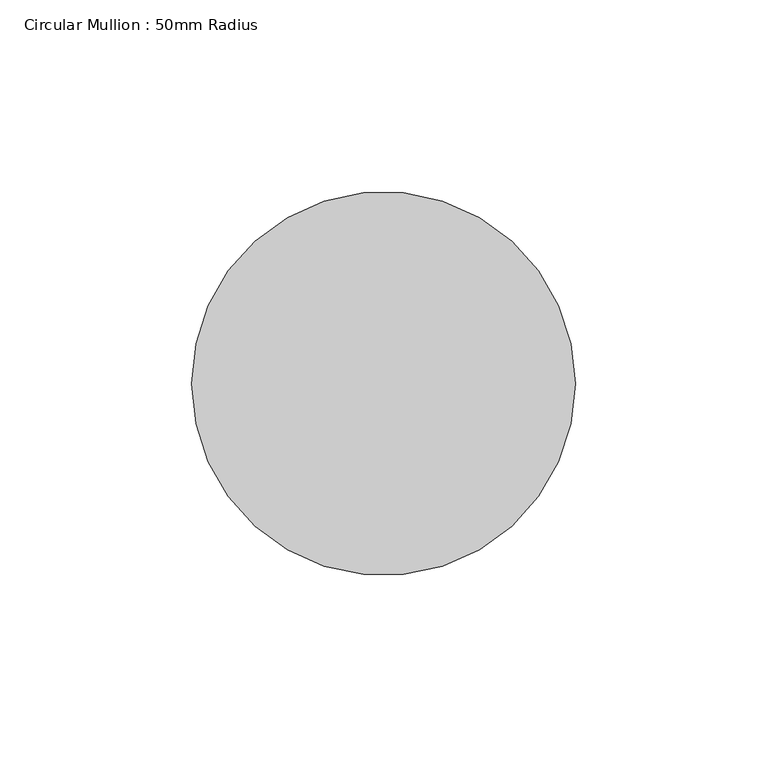
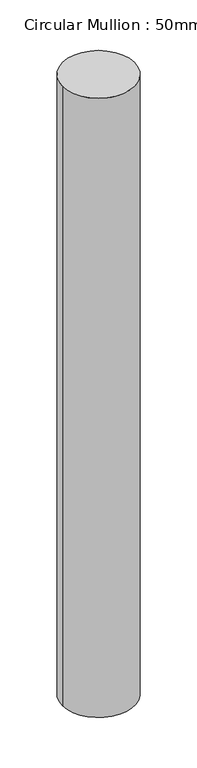
"""IFC4 building model written with IfcOpenShell, lengths in millimetres: member geometry, Circular Mullion : 50mm Radius."""

import ifcopenshell
import ifcopenshell.guid

model = None  # the IFC model being written
_history = None  # IfcOwnerHistory: only IFC2X3 demands one
_inside = {}  # id of a spatial element -> (the spatial element, [elements in it])
_under = {}  # id of a project, library or spatial element -> (it, [spatial elements below it])
_declared = {}  # id of a project -> (the project, [libraries it declares])
_typed = {}  # id of a type object -> (the type object, [elements of that type])
_made_of = {}  # id of a material, layer set ... -> (it, [elements and type objects made of it])


def new_model(schema):
    """Start an empty IFC model of exactly this schema.

    Asked for "IFC4X3", IfcOpenShell would pick the latest addendum, in which some entities
    have other attributes; the version numbers below select the first issue.
    IFC2X3 requires an IfcOwnerHistory on every rooted entity: one is made here for all.
    """
    global model, _history
    if schema == "IFC4X3":
        model = ifcopenshell.file(schema_version=(4, 3, 0, 0))
    else:
        model = ifcopenshell.file(schema=schema)
    _inside.clear()
    _under.clear()
    _declared.clear()
    _typed.clear()
    _made_of.clear()
    _history = None
    if model.schema == "IFC2X3":
        org = make("IfcOrganization", Name="unknown")
        user = make(
            "IfcPersonAndOrganization",
            ThePerson=make("IfcPerson", FamilyName="unknown"),
            TheOrganization=org,
        )
        app = make(
            "IfcApplication",
            ApplicationDeveloper=org,
            Version="unknown",
            ApplicationFullName="unknown",
            ApplicationIdentifier="unknown",
        )
        _history = make(
            "IfcOwnerHistory",
            OwningUser=user,
            OwningApplication=app,
            ChangeAction="ADDED",
            CreationDate=0,
        )
    return model


def make(cls, **values):
    """One entity of the class cls with the attributes given. An attribute that is None is left unset."""
    return model.create_entity(
        cls, **{name: value for name, value in values.items() if value is not None}
    )


def rooted(cls, **values):
    """An entity with a GlobalId (a new one), such as an element, a storey or a relation."""
    return make(cls, GlobalId=ifcopenshell.guid.new(), OwnerHistory=_history, **values)


def si_unit(unit_type, name, prefix=None):
    """IfcSIUnit, for example si_unit("LENGTHUNIT", "METRE", prefix="MILLI")."""
    return make("IfcSIUnit", UnitType=unit_type, Prefix=prefix, Name=name)


def assignment(units):
    """IfcUnitAssignment: the units of a project."""
    return None if units is None else make("IfcUnitAssignment", Units=units)


def point(xyz):
    """IfcCartesianPoint."""
    return None if xyz is None else make("IfcCartesianPoint", Coordinates=xyz)


def direction(xyz):
    """IfcDirection."""
    return None if xyz is None else make("IfcDirection", DirectionRatios=xyz)


def frame(location, z_axis=None, x_axis=None):
    """IfcAxis2Placement3D, a coordinate frame: its origin and axes. An axis left out is left unset."""
    return make(
        "IfcAxis2Placement3D",
        Location=point(location),
        Axis=direction(z_axis),
        RefDirection=direction(x_axis),
    )


def frame_2d(location, x_axis=None):
    """IfcAxis2Placement2D, a coordinate frame in the plane: its origin and x axis."""
    return make(
        "IfcAxis2Placement2D", Location=point(location), RefDirection=direction(x_axis)
    )


def origin():
    """The frame at (0, 0, 0) with its axes left unset."""
    return frame((0.0, 0.0, 0.0))


def origin_2d():
    """The frame at (0, 0) in the plane with its x axis left unset."""
    return frame_2d((0.0, 0.0))


def place(relative_to, where):
    """IfcLocalPlacement: puts the frame where relative to a parent placement (None: the world)."""
    return make(
        "IfcLocalPlacement", PlacementRelTo=relative_to, RelativePlacement=where
    )


def context(
    kind, dimensions, precision=None, world=None, true_north=None, identifier=None
):
    """IfcGeometricRepresentationContext, for example the 3D "Model" context."""
    return make(
        "IfcGeometricRepresentationContext",
        ContextIdentifier=identifier,
        ContextType=kind,
        CoordinateSpaceDimension=dimensions,
        Precision=precision,
        WorldCoordinateSystem=world,
        TrueNorth=true_north,
    )


def project(units=None, contexts=None):
    """IfcProject with its units and contexts."""
    return rooted(
        "IfcProject",
        Name="project",
        RepresentationContexts=contexts,
        UnitsInContext=assignment(units),
    )


def spatial(cls, under=None, at=None, **own):
    """A site, building, storey or space (cls), placed at a placement, below another one or the project."""
    s = rooted(cls, ObjectPlacement=at, **own)
    if under is not None:
        _under.setdefault(under.id(), (under, []))[1].append(s)
    return s


def circle_curve(where, radius):
    """IfcCircle in the frame where."""
    return make("IfcCircle", Position=where, Radius=radius)


def trimmed(basis, trim1, trim2, sense, master):
    """IfcTrimmedCurve: the piece of a basis curve between two trims."""
    return make(
        "IfcTrimmedCurve",
        BasisCurve=basis,
        Trim1=trim1,
        Trim2=trim2,
        SenseAgreement=sense,
        MasterRepresentation=master,
    )


def segment(curve, same_sense, transition):
    """IfcCompositeCurveSegment."""
    return make(
        "IfcCompositeCurveSegment",
        Transition=transition,
        SameSense=same_sense,
        ParentCurve=curve,
    )


def composite_curve(segments, self_intersect=None):
    """IfcCompositeCurve: segments joined end to end."""
    return make("IfcCompositeCurve", Segments=segments, SelfIntersect=self_intersect)


def outline(outer, holes=None, kind="AREA"):
    """IfcArbitraryClosedProfileDef: a profile drawn as a closed curve; with holes, ...WithVoids."""
    if holes is None:
        return make("IfcArbitraryClosedProfileDef", ProfileType=kind, OuterCurve=outer)
    return make(
        "IfcArbitraryProfileDefWithVoids",
        ProfileType=kind,
        OuterCurve=outer,
        InnerCurves=holes,
    )


def extrude(swept, where, along, depth):
    """IfcExtrudedAreaSolid: the profile swept, set in the frame where, extruded along a direction by depth."""
    return make(
        "IfcExtrudedAreaSolid",
        SweptArea=swept,
        Position=where,
        ExtrudedDirection=direction(along),
        Depth=depth,
    )


def shape(context_of_items, identifier, shape_type, items):
    """IfcShapeRepresentation: the items that make up one representation, for example the "Body"."""
    return make(
        "IfcShapeRepresentation",
        ContextOfItems=context_of_items,
        RepresentationIdentifier=identifier,
        RepresentationType=shape_type,
        Items=items,
    )


def source(mapping_origin, context_of_items, identifier, shape_type, items):
    """IfcRepresentationMap: a shape defined once, which mapped items show again and again."""
    return make(
        "IfcRepresentationMap",
        MappingOrigin=mapping_origin,
        MappedRepresentation=shape(context_of_items, identifier, shape_type, items),
    )


def transform(
    local_origin,
    x_axis=None,
    y_axis=None,
    z_axis=None,
    scale=None,
    scale2=None,
    scale3=None,
    uniform=True,
):
    """IfcCartesianTransformationOperator3D, or its non-uniform kind. x_axis, y_axis, z_axis: its Axis1, 2, 3."""
    if uniform:
        return make(
            "IfcCartesianTransformationOperator3D",
            Axis1=direction(x_axis),
            Axis2=direction(y_axis),
            LocalOrigin=point(local_origin),
            Scale=scale,
            Axis3=direction(z_axis),
        )
    return make(
        "IfcCartesianTransformationOperator3DnonUniform",
        Axis1=direction(x_axis),
        Axis2=direction(y_axis),
        LocalOrigin=point(local_origin),
        Scale=scale,
        Axis3=direction(z_axis),
        Scale2=scale2,
        Scale3=scale3,
    )


def mapped(mapping_source, mapping_target):
    """IfcMappedItem: shows the shape of a source again, moved by a transform."""
    return make(
        "IfcMappedItem", MappingSource=mapping_source, MappingTarget=mapping_target
    )


def made_of(thing, what):
    """Note that an element or type object is made of a material, layer set ...; save() writes the relation."""
    if what is not None:
        _made_of.setdefault(what.id(), (what, []))[1].append(thing)
    return thing


def element(
    cls,
    number,
    at=None,
    inside=None,
    cuts=None,
    type_object=None,
    material=None,
    context=None,
    identifier="Body",
    shape_type=None,
    held_by="IfcProductDefinitionShape",
    body=None,
    shapes=None,
    **own,
):
    """One element of the class cls, such as IfcWall. Its Tag is "e" and its number.

    at: its placement. inside: the storey or other place that contains it. cuts: it is an
    opening in that element (IfcRelVoidsElement). A single representation is given by context,
    identifier, shape_type and body (its items); several are given by shapes. held_by: the class
    of the entity that holds the representations. save() writes the other relations.
    """
    e = rooted(cls, Tag="e%d" % number, ObjectPlacement=at, **own)
    if body is not None:
        shapes = [shape(context, identifier, shape_type, body)]
    if shapes is not None:
        e.Representation = make(held_by, Representations=shapes)
    if inside is not None:
        _inside.setdefault(inside.id(), (inside, []))[1].append(e)
    if cuts is not None:
        rooted(
            "IfcRelVoidsElement", RelatingBuildingElement=cuts, RelatedOpeningElement=e
        )
    if type_object is not None:
        _typed.setdefault(type_object.id(), (type_object, []))[1].append(e)
    return made_of(e, material)


def aggregate(whole, parts):
    """IfcRelAggregates: a whole, such as a stair, and the parts it consists of."""
    return rooted("IfcRelAggregates", RelatingObject=whole, RelatedObjects=parts)


def save(model, path):
    """Write the relations noted so far, then the file.

    IfcRelAggregates (storeys below a building ...), IfcRelContainedInSpatialStructure (elements
    in a storey), IfcRelDefinesByType, IfcRelAssociatesMaterial and IfcRelDeclares: one each for
    every whole, place, type object, material and project.
    """
    for whole, parts in _under.values():
        aggregate(whole, parts)
    for where, things in _inside.values():
        rooted(
            "IfcRelContainedInSpatialStructure",
            RelatedElements=things,
            RelatingStructure=where,
        )
    for kind, things in _typed.values():
        rooted("IfcRelDefinesByType", RelatedObjects=things, RelatingType=kind)
    for what, things in _made_of.values():
        rooted("IfcRelAssociatesMaterial", RelatedObjects=things, RelatingMaterial=what)
    for by, libraries in _declared.values():
        rooted("IfcRelDeclares", RelatingContext=by, RelatedDefinitions=libraries)
    model.write(path)


def circular_mullion_50mm_radius_f52ad554(model_context):
    return source(origin(), model_context, "Body", "SweptSolid", [
        extrude(outline(composite_curve([segment(trimmed(circle_curve(origin_2d(), 50.0), [point((50.0, 0.0))], [point((-50.0, 0.0))], False, "CARTESIAN"), True, "CONTINUOUS"), segment(trimmed(circle_curve(origin_2d(), 50.0), [point((-50.0, 0.0))], [point((50.0, 0.0))], False, "CARTESIAN"), True, "CONTINUOUS")], self_intersect=False)), frame((0.0, 0.0, -905.7222099), z_axis=(0.0, 0.0, 1.0), x_axis=(1.0, 0.0, 0.0)), (0.0, 0.0, 1.0), 905.7222099),
    ])


if __name__ == "__main__":
    model = new_model("IFC4")
    model_context = context("Model", 3, world=origin())
    ifc_project = project(units=[si_unit("LENGTHUNIT", "METRE", prefix="MILLI")], contexts=[model_context])
    site = spatial("IfcSite", under=ifc_project)
    building = spatial("IfcBuilding", under=site)
    placement = place(None, origin())
    circular_mullion_50mm_radius_shape = circular_mullion_50mm_radius_f52ad554(model_context)
    element("IfcMember", 1, ObjectType="Circular Mullion : 50mm Radius", at=placement, inside=building, context=model_context, shape_type="MappedRepresentation", body=[
        mapped(circular_mullion_50mm_radius_shape, transform((0.0, 0.0, 0.0), x_axis=(1.0, 0.0, 0.0), y_axis=(0.0, 1.0, 0.0), z_axis=(0.0, 0.0, 1.0))),
    ])
    save(model, "model.ifc")

# Revit data of these elements
# Type "Circular Mullion : 50mm Radius"
#   built-in parameter 1007350 = 0.164042 (stored number, unit not read)
# Element 1 (IfcMember, "Circular Mullion : 50mm Radius")
#   Materials on its faces: "Aluminium"
# Materials
#   "Aluminium": class "Metal", colour RGB 247 247 247, transparency 0, Description = "Aluminium 6061", Cost = 0
